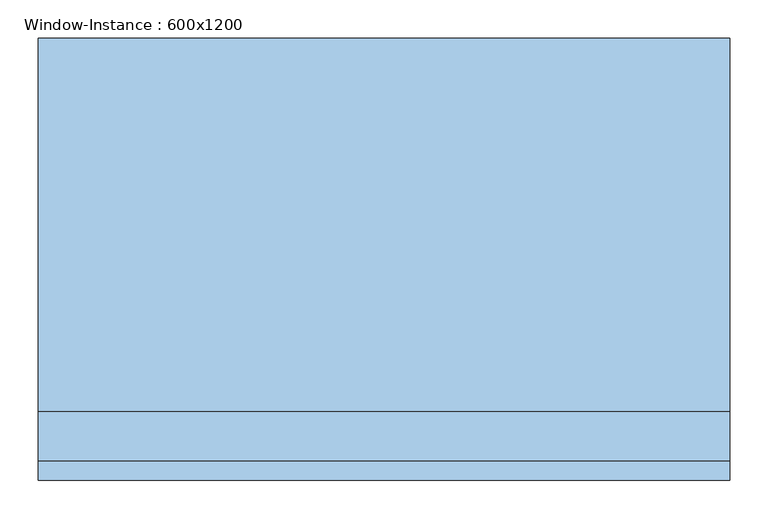
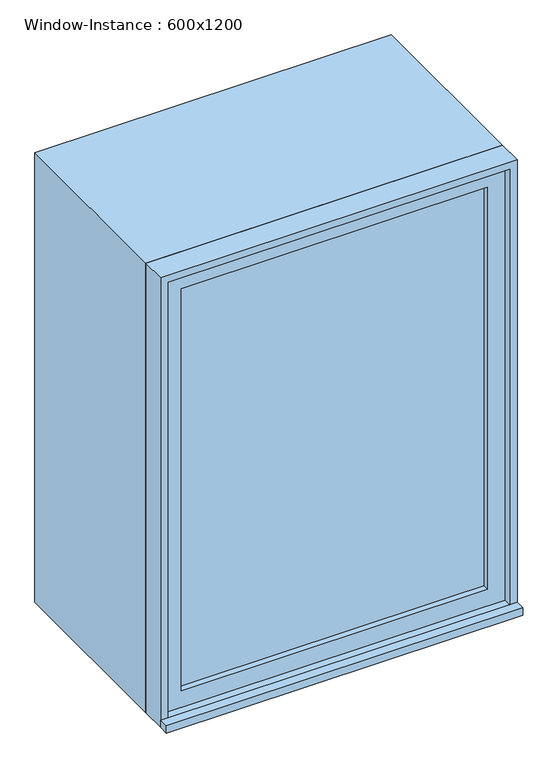
"""IFC4 building model written with IfcOpenShell, lengths in millimetres: window geometry, Window-Instance : 600x1200."""

import ifcopenshell
import ifcopenshell.guid

model = None  # the IFC model being written
_history = None  # IfcOwnerHistory: only IFC2X3 demands one
_inside = {}  # id of a spatial element -> (the spatial element, [elements in it])
_under = {}  # id of a project, library or spatial element -> (it, [spatial elements below it])
_declared = {}  # id of a project -> (the project, [libraries it declares])
_typed = {}  # id of a type object -> (the type object, [elements of that type])
_made_of = {}  # id of a material, layer set ... -> (it, [elements and type objects made of it])


def new_model(schema):
    """Start an empty IFC model of exactly this schema.

    Asked for "IFC4X3", IfcOpenShell would pick the latest addendum, in which some entities
    have other attributes; the version numbers below select the first issue.
    IFC2X3 requires an IfcOwnerHistory on every rooted entity: one is made here for all.
    """
    global model, _history
    if schema == "IFC4X3":
        model = ifcopenshell.file(schema_version=(4, 3, 0, 0))
    else:
        model = ifcopenshell.file(schema=schema)
    _inside.clear()
    _under.clear()
    _declared.clear()
    _typed.clear()
    _made_of.clear()
    _history = None
    if model.schema == "IFC2X3":
        org = make("IfcOrganization", Name="unknown")
        user = make(
            "IfcPersonAndOrganization",
            ThePerson=make("IfcPerson", FamilyName="unknown"),
            TheOrganization=org,
        )
        app = make(
            "IfcApplication",
            ApplicationDeveloper=org,
            Version="unknown",
            ApplicationFullName="unknown",
            ApplicationIdentifier="unknown",
        )
        _history = make(
            "IfcOwnerHistory",
            OwningUser=user,
            OwningApplication=app,
            ChangeAction="ADDED",
            CreationDate=0,
        )
    return model


def make(cls, **values):
    """One entity of the class cls with the attributes given. An attribute that is None is left unset."""
    return model.create_entity(
        cls, **{name: value for name, value in values.items() if value is not None}
    )


def rooted(cls, **values):
    """An entity with a GlobalId (a new one), such as an element, a storey or a relation."""
    return make(cls, GlobalId=ifcopenshell.guid.new(), OwnerHistory=_history, **values)


def si_unit(unit_type, name, prefix=None):
    """IfcSIUnit, for example si_unit("LENGTHUNIT", "METRE", prefix="MILLI")."""
    return make("IfcSIUnit", UnitType=unit_type, Prefix=prefix, Name=name)


def assignment(units):
    """IfcUnitAssignment: the units of a project."""
    return None if units is None else make("IfcUnitAssignment", Units=units)


def point(xyz):
    """IfcCartesianPoint."""
    return None if xyz is None else make("IfcCartesianPoint", Coordinates=xyz)


def direction(xyz):
    """IfcDirection."""
    return None if xyz is None else make("IfcDirection", DirectionRatios=xyz)


def frame(location, z_axis=None, x_axis=None):
    """IfcAxis2Placement3D, a coordinate frame: its origin and axes. An axis left out is left unset."""
    return make(
        "IfcAxis2Placement3D",
        Location=point(location),
        Axis=direction(z_axis),
        RefDirection=direction(x_axis),
    )


def origin():
    """The frame at (0, 0, 0) with its axes left unset."""
    return frame((0.0, 0.0, 0.0))


def place(relative_to, where):
    """IfcLocalPlacement: puts the frame where relative to a parent placement (None: the world)."""
    return make(
        "IfcLocalPlacement", PlacementRelTo=relative_to, RelativePlacement=where
    )


def context(
    kind, dimensions, precision=None, world=None, true_north=None, identifier=None
):
    """IfcGeometricRepresentationContext, for example the 3D "Model" context."""
    return make(
        "IfcGeometricRepresentationContext",
        ContextIdentifier=identifier,
        ContextType=kind,
        CoordinateSpaceDimension=dimensions,
        Precision=precision,
        WorldCoordinateSystem=world,
        TrueNorth=true_north,
    )


def project(units=None, contexts=None):
    """IfcProject with its units and contexts."""
    return rooted(
        "IfcProject",
        Name="project",
        RepresentationContexts=contexts,
        UnitsInContext=assignment(units),
    )


def spatial(cls, under=None, at=None, **own):
    """A site, building, storey or space (cls), placed at a placement, below another one or the project."""
    s = rooted(cls, ObjectPlacement=at, **own)
    if under is not None:
        _under.setdefault(under.id(), (under, []))[1].append(s)
    return s


def polyline(points):
    """IfcPolyline through the points."""
    return make("IfcPolyline", Points=[point(p) for p in points])


def outline(outer, holes=None, kind="AREA"):
    """IfcArbitraryClosedProfileDef: a profile drawn as a closed curve; with holes, ...WithVoids."""
    if holes is None:
        return make("IfcArbitraryClosedProfileDef", ProfileType=kind, OuterCurve=outer)
    return make(
        "IfcArbitraryProfileDefWithVoids",
        ProfileType=kind,
        OuterCurve=outer,
        InnerCurves=holes,
    )


def extrude(swept, where, along, depth):
    """IfcExtrudedAreaSolid: the profile swept, set in the frame where, extruded along a direction by depth."""
    return make(
        "IfcExtrudedAreaSolid",
        SweptArea=swept,
        Position=where,
        ExtrudedDirection=direction(along),
        Depth=depth,
    )


def shape(context_of_items, identifier, shape_type, items):
    """IfcShapeRepresentation: the items that make up one representation, for example the "Body"."""
    return make(
        "IfcShapeRepresentation",
        ContextOfItems=context_of_items,
        RepresentationIdentifier=identifier,
        RepresentationType=shape_type,
        Items=items,
    )


def source(mapping_origin, context_of_items, identifier, shape_type, items):
    """IfcRepresentationMap: a shape defined once, which mapped items show again and again."""
    return make(
        "IfcRepresentationMap",
        MappingOrigin=mapping_origin,
        MappedRepresentation=shape(context_of_items, identifier, shape_type, items),
    )


def transform(
    local_origin,
    x_axis=None,
    y_axis=None,
    z_axis=None,
    scale=None,
    scale2=None,
    scale3=None,
    uniform=True,
):
    """IfcCartesianTransformationOperator3D, or its non-uniform kind. x_axis, y_axis, z_axis: its Axis1, 2, 3."""
    if uniform:
        return make(
            "IfcCartesianTransformationOperator3D",
            Axis1=direction(x_axis),
            Axis2=direction(y_axis),
            LocalOrigin=point(local_origin),
            Scale=scale,
            Axis3=direction(z_axis),
        )
    return make(
        "IfcCartesianTransformationOperator3DnonUniform",
        Axis1=direction(x_axis),
        Axis2=direction(y_axis),
        LocalOrigin=point(local_origin),
        Scale=scale,
        Axis3=direction(z_axis),
        Scale2=scale2,
        Scale3=scale3,
    )


def mapped(mapping_source, mapping_target):
    """IfcMappedItem: shows the shape of a source again, moved by a transform."""
    return make(
        "IfcMappedItem", MappingSource=mapping_source, MappingTarget=mapping_target
    )


def made_of(thing, what):
    """Note that an element or type object is made of a material, layer set ...; save() writes the relation."""
    if what is not None:
        _made_of.setdefault(what.id(), (what, []))[1].append(thing)
    return thing


def element(
    cls,
    number,
    at=None,
    inside=None,
    cuts=None,
    type_object=None,
    material=None,
    context=None,
    identifier="Body",
    shape_type=None,
    held_by="IfcProductDefinitionShape",
    body=None,
    shapes=None,
    **own,
):
    """One element of the class cls, such as IfcWall. Its Tag is "e" and its number.

    at: its placement. inside: the storey or other place that contains it. cuts: it is an
    opening in that element (IfcRelVoidsElement). A single representation is given by context,
    identifier, shape_type and body (its items); several are given by shapes. held_by: the class
    of the entity that holds the representations. save() writes the other relations.
    """
    e = rooted(cls, Tag="e%d" % number, ObjectPlacement=at, **own)
    if body is not None:
        shapes = [shape(context, identifier, shape_type, body)]
    if shapes is not None:
        e.Representation = make(held_by, Representations=shapes)
    if inside is not None:
        _inside.setdefault(inside.id(), (inside, []))[1].append(e)
    if cuts is not None:
        rooted(
            "IfcRelVoidsElement", RelatingBuildingElement=cuts, RelatedOpeningElement=e
        )
    if type_object is not None:
        _typed.setdefault(type_object.id(), (type_object, []))[1].append(e)
    return made_of(e, material)


def aggregate(whole, parts):
    """IfcRelAggregates: a whole, such as a stair, and the parts it consists of."""
    return rooted("IfcRelAggregates", RelatingObject=whole, RelatedObjects=parts)


def save(model, path):
    """Write the relations noted so far, then the file.

    IfcRelAggregates (storeys below a building ...), IfcRelContainedInSpatialStructure (elements
    in a storey), IfcRelDefinesByType, IfcRelAssociatesMaterial and IfcRelDeclares: one each for
    every whole, place, type object, material and project.
    """
    for whole, parts in _under.values():
        aggregate(whole, parts)
    for where, things in _inside.values():
        rooted(
            "IfcRelContainedInSpatialStructure",
            RelatedElements=things,
            RelatingStructure=where,
        )
    for kind, things in _typed.values():
        rooted("IfcRelDefinesByType", RelatedObjects=things, RelatingType=kind)
    for what, things in _made_of.values():
        rooted("IfcRelAssociatesMaterial", RelatedObjects=things, RelatingMaterial=what)
    for by, libraries in _declared.values():
        rooted("IfcRelDeclares", RelatingContext=by, RelatedDefinitions=libraries)
    model.write(path)


def window_instance_600x1200_939708ca(model_context):
    return source(origin(), model_context, "Body", "SweptSolid", [
        extrude(outline(polyline([(-488.1, -300.4), (-488.1, -275.0), (411.9, -275.0), (411.9, -300.4), (-488.1, -300.4)])), frame((0.0, 0.0, 900.0), z_axis=(0.0, 0.0, 1.0), x_axis=(1.0, 0.0, 0.0)), (0.0, 0.0, 1.0), 19.05),
        extrude(outline(polyline([(348.4, -226.425), (348.4, -239.125), (-424.6, -239.125), (-424.6, -226.425), (348.4, -226.425)])), frame((0.0, 0.0, 963.5), z_axis=(0.0, 0.0, 1.0), x_axis=(1.0, 0.0, 0.0)), (0.0, 0.0, 1.0), 1073.0),
        extrude(outline(polyline([(2080.95, -469.05), (919.05, -469.05), (919.05, 392.85), (2080.95, 392.85), (2080.95, -469.05)]), holes=[polyline([(2036.5, -424.6), (2036.5, 348.4), (963.5, 348.4), (963.5, -424.6), (2036.5, -424.6)])]), frame((0.0, -255.0, 0.0), z_axis=(0.0, 1.0, 0.0), x_axis=(0.0, 0.0, 1.0)), (0.0, 0.0, 1.0), 44.45),
        extrude(outline(polyline([(2100.0, -488.1), (900.0, -488.1), (900.0, 411.9), (2100.0, 411.9), (2100.0, -488.1)]), holes=[polyline([(2068.25, -456.35), (2068.25, 380.15), (931.75, 380.15), (931.75, -456.35), (2068.25, -456.35)])]), frame((0.0, -210.55, 0.0), z_axis=(0.0, 1.0, 0.0), x_axis=(0.0, 0.0, 1.0)), (0.0, 0.0, 1.0), 485.55),
        extrude(outline(polyline([(2100.0, 411.9), (2100.0, -488.1), (900.0, -488.1), (900.0, 411.9), (2100.0, 411.9)]), holes=[polyline([(2080.95, 392.85), (919.05, 392.85), (919.05, -469.05), (2080.95, -469.05), (2080.95, 392.85)])]), frame((0.0, -275.0, 0.0), z_axis=(0.0, 1.0, 0.0), x_axis=(0.0, 0.0, 1.0)), (0.0, 0.0, 1.0), 64.45),
    ])


if __name__ == "__main__":
    model = new_model("IFC4")
    model_context = context("Model", 3, world=origin())
    ifc_project = project(units=[si_unit("LENGTHUNIT", "METRE", prefix="MILLI")], contexts=[model_context])
    site = spatial("IfcSite", under=ifc_project)
    building = spatial("IfcBuilding", under=site)
    placement = place(None, origin())
    window_instance_600x1200_shape = window_instance_600x1200_939708ca(model_context)
    element("IfcWindow", 1, ObjectType="Window-Instance : 600x1200", at=placement, inside=building, context=model_context, shape_type="MappedRepresentation", body=[
        mapped(window_instance_600x1200_shape, transform((0.0, 0.0, 0.0), x_axis=(1.0, 0.0, 0.0), y_axis=(0.0, 1.0, 0.0), z_axis=(0.0, 0.0, 1.0))),
    ])
    save(model, "model.ifc")

# Revit data of these elements
# Type "Window-Instance : 600x1200"
#   Type Mark = "7"
#   Construction Type Id = "GSP4R"
#   Assembly Code = "B2020100"
#   Analytic Construction = "1/8 in Pilkington single glazing"
#   Visual Light Transmittance = 0.9
#   Thermal Resistance (R) = 0.149095 (m²·K)/W
#   Solar Heat Gain Coefficient = 0.86
#   Heat Transfer Coefficient (U) = 6.70716 W/(m²·K)
#   Height [instance default] = 1200 mm
#   Default Sill Height = 900 mm
#   Width [instance default] = 600 mm
#   Window Inset = 20 mm
#   Glass Pane Material = WW-EC-GL-Storefront
#   Sash Material = WW-EC-RGB-White
#   Wall Closure = (empty or 0)
# Element 1 (IfcWindow, "Window-Instance : 600x1200")
#   Width = 900 mm
#   Materials on its faces: "WW-EC-RGB-White", "WW-EC-GL-Storefront"
# Materials
#   "WW-EC-GL-Storefront": class "Glass", colour RGB 236 240 239, transparency 0.85, Description = "Storefront Glass", Cost = 0
#   "WW-EC-RGB-White": class "Generic", colour RGB 255 255 255, transparency 0, Comments = "If region requests off-white, swith asset color to RGB 231-228-220", Description = "Generic Color", Cost = 0
